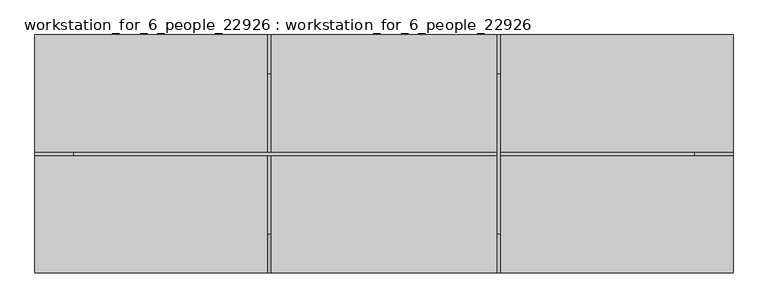
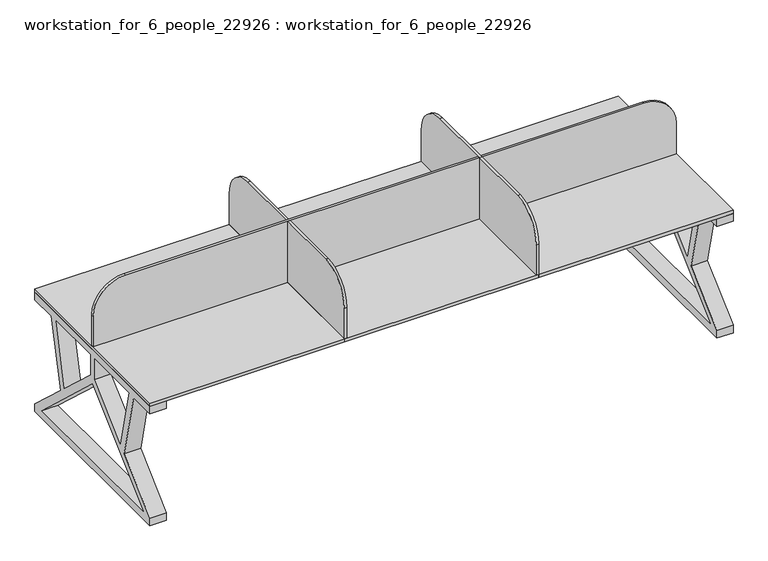
"""IFC4 building model written with IfcOpenShell, lengths in millimetres: proxy geometry, workstation_for_6_people_22926 : workstation_for_6_people_22926."""

from ifc_helpers import new_model, si_unit, point, frame, frame_2d, origin, place, context, project, spatial, polyline, circle_curve, trimmed, segment, composite_curve, outline, extrude, source, transform, mapped, element, save


def workstation_for_6_people_22926_workstation_for_6_people_fb55f467(model_context):
    return source(origin(), model_context, "Body", "SweptSolid", [
        extrude(outline(polyline([(600.0, 615.0), (600.0, -615.0), (-600.0, -615.0), (-600.0, 615.0), (600.0, 615.0)])), frame((0.0, 0.0, 780.0), z_axis=(0.0, 0.0, 1.0), x_axis=(1.0, 0.0, 0.0)), (0.0, 0.0, 1.0), 20.0),
        extrude(outline(polyline([(1800.0, 615.0), (1800.0, -615.0), (600.0, -615.0), (600.0, 615.0), (1800.0, 615.0)])), frame((0.0, 0.0, 780.0), z_axis=(0.0, 0.0, 1.0), x_axis=(1.0, 0.0, 0.0)), (0.0, 0.0, 1.0), 20.0),
        extrude(outline(polyline([(3000.0, 615.0), (3000.0, -615.0), (1800.0, -615.0), (1800.0, 615.0), (3000.0, 615.0)])), frame((0.0, 0.0, 780.0), z_axis=(0.0, 0.0, 1.0), x_axis=(1.0, 0.0, 0.0)), (0.0, 0.0, 1.0), 20.0),
        extrude(outline(composite_curve([segment(polyline([(-415.0, 1200.0), (415.0, 1200.0)]), True, "CONTINUOUS"), segment(trimmed(circle_curve(frame_2d((415.0, 1000.0)), 200.0), [point((415.0, 1200.0))], [point((615.0, 1000.0))], False, "CARTESIAN"), True, "CONTINUOUS"), segment(polyline([(615.0, 1000.0), (615.0, 800.0), (-615.0, 800.0), (-615.0, 1000.0)]), True, "CONTINUOUS"), segment(trimmed(circle_curve(frame_2d((-415.0, 1000.0)), 200.0), [point((-615.0, 1000.0))], [point((-415.0, 1200.0))], False, "CARTESIAN"), True, "CONTINUOUS")], self_intersect=False)), frame((1785.0, 0.0, 0.0), z_axis=(1.0, 0.0, 0.0), x_axis=(0.0, 1.0, 0.0)), (0.0, 0.0, 1.0), 15.0),
        extrude(outline(composite_curve([segment(polyline([(-415.0, 1200.0), (415.0, 1200.0)]), True, "CONTINUOUS"), segment(trimmed(circle_curve(frame_2d((415.0, 1000.0)), 200.0), [point((415.0, 1200.0))], [point((615.0, 1000.0))], False, "CARTESIAN"), True, "CONTINUOUS"), segment(polyline([(615.0, 1000.0), (615.0, 800.0), (-615.0, 800.0), (-615.0, 1000.0)]), True, "CONTINUOUS"), segment(trimmed(circle_curve(frame_2d((-415.0, 1000.0)), 200.0), [point((-615.0, 1000.0))], [point((-415.0, 1200.0))], False, "CARTESIAN"), True, "CONTINUOUS")], self_intersect=False)), frame((1785.0, 0.0, 0.0), z_axis=(1.0, 0.0, 0.0), x_axis=(0.0, 1.0, 0.0)), (0.0, 0.0, 1.0), 15.0),
        extrude(outline(composite_curve([segment(polyline([(1200.0, 2800.0), (1200.0, -400.0)]), True, "CONTINUOUS"), segment(trimmed(circle_curve(frame_2d((1000.0, -400.0)), 200.0), [point((1200.0, -400.0))], [point((1000.0, -600.0))], False, "CARTESIAN"), True, "CONTINUOUS"), segment(polyline([(1000.0, -600.0), (800.0, -600.0), (800.0, 3000.0), (1000.0, 3000.0)]), True, "CONTINUOUS"), segment(trimmed(circle_curve(frame_2d((1000.0, 2800.0)), 200.0), [point((1000.0, 3000.0))], [point((1200.0, 2800.0))], False, "CARTESIAN"), True, "CONTINUOUS")], self_intersect=False)), frame((0.0, -7.5, 0.0), z_axis=(0.0, 1.0, 0.0), x_axis=(0.0, 0.0, 1.0)), (0.0, 0.0, 1.0), 15.0),
        extrude(outline(polyline([(615.0, 0.0), (-615.0, 0.0), (-615.0, 50.0), (-341.0964873, 304.1731749), (-440.6744526, 730.0), (-615.0, 730.0), (-615.0, 780.0), (615.0, 780.0), (615.0, 730.0), (440.6744526, 730.0), (341.0964873, 304.1731749), (615.0, 50.0), (615.0, 0.0)]), holes=[polyline([(541.4935909, 50.0), (0.0, 552.4876967), (-541.4935909, 50.0), (541.4935909, 50.0)]), polyline([(-298.9035127, 343.3268251), (-25.0, 597.5), (-25.0, 730.0), (-389.3255474, 730.0), (-298.9035127, 343.3268251)]), polyline([(298.9035127, 343.3268251), (389.3255474, 730.0), (25.0, 730.0), (25.0, 597.5), (298.9035127, 343.3268251)])]), frame((2900.0, 0.0, 0.0), z_axis=(1.0, 0.0, 0.0), x_axis=(0.0, 1.0, 0.0)), (0.0, 0.0, 1.0), 100.0),
        extrude(outline(polyline([(615.0, 0.0), (-615.0, 0.0), (-615.0, 50.0), (-341.0964873, 304.1731749), (-440.6744526, 730.0), (-615.0, 730.0), (-615.0, 780.0), (615.0, 780.0), (615.0, 730.0), (440.6744526, 730.0), (341.0964873, 304.1731749), (615.0, 50.0), (615.0, 0.0)]), holes=[polyline([(541.4935909, 50.0), (0.0, 552.4876967), (-541.4935909, 50.0), (541.4935909, 50.0)]), polyline([(-298.9035127, 343.3268251), (-25.0, 597.5), (-25.0, 730.0), (-389.3255474, 730.0), (-298.9035127, 343.3268251)]), polyline([(298.9035127, 343.3268251), (389.3255474, 730.0), (25.0, 730.0), (25.0, 597.5), (298.9035127, 343.3268251)])]), frame((-600.0, 0.0, 0.0), z_axis=(1.0, 0.0, 0.0), x_axis=(0.0, 1.0, 0.0)), (0.0, 0.0, 1.0), 100.0),
        extrude(outline(composite_curve([segment(polyline([(-415.0, 1200.0), (415.0, 1200.0)]), True, "CONTINUOUS"), segment(trimmed(circle_curve(frame_2d((415.0, 1000.0)), 200.0), [point((415.0, 1200.0))], [point((615.0, 1000.0))], False, "CARTESIAN"), True, "CONTINUOUS"), segment(polyline([(615.0, 1000.0), (615.0, 800.0), (-615.0, 800.0), (-615.0, 1000.0)]), True, "CONTINUOUS"), segment(trimmed(circle_curve(frame_2d((-415.0, 1000.0)), 200.0), [point((-615.0, 1000.0))], [point((-415.0, 1200.0))], False, "CARTESIAN"), True, "CONTINUOUS")], self_intersect=False)), frame((600.0, 0.0, 0.0), z_axis=(1.0, 0.0, 0.0), x_axis=(0.0, 1.0, 0.0)), (0.0, 0.0, 1.0), 15.0),
    ])


if __name__ == "__main__":
    model = new_model("IFC4")
    model_context = context("Model", 3, world=origin())
    ifc_project = project(units=[si_unit("LENGTHUNIT", "METRE", prefix="MILLI")], contexts=[model_context])
    site = spatial("IfcSite", under=ifc_project)
    building = spatial("IfcBuilding", under=site)
    placement = place(None, origin())
    workstation_for_6_people_22926_workstation_for_6_people_shape = workstation_for_6_people_22926_workstation_for_6_people_fb55f467(model_context)
    element("IfcBuildingElementProxy", 1, Name="workstation_for_6_people_22926 : workstation_for_6_people_22926", ObjectType="workstation_for_6_people_22926 : workstation_for_6_people_22926", at=placement, inside=building, context=model_context, shape_type="MappedRepresentation", body=[
        mapped(workstation_for_6_people_22926_workstation_for_6_people_shape, transform((0.0, 0.0, 0.0), x_axis=(1.0, 0.0, 0.0), y_axis=(0.0, 1.0, 0.0), z_axis=(0.0, 0.0, 1.0))),
    ])
    save(model, "model.ifc")

# Revit data of these elements
# Type "workstation_for_6_people_22926 : workstation_for_6_people_22926"
#   Default Elevation = 0
# Element 1 (IfcBuildingElementProxy, "workstation_for_6_people_22926 : workstation_for_6_people_22926")
#   Materials on its faces: "white", "green"
# Materials
#   "white": class "Generic", colour RGB 219 219 219, transparency 0, Cost = 0
#   "green": class "Generic", colour RGB 0 255 127, transparency 0, Cost = 0
